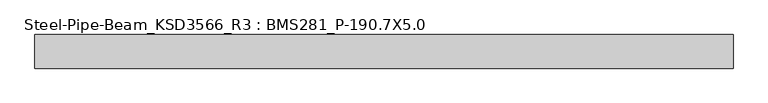
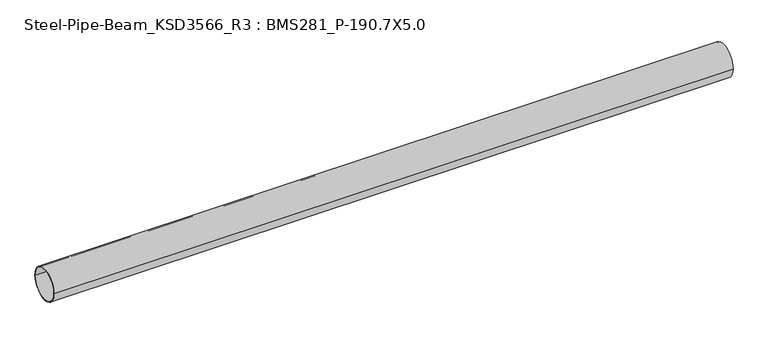
"""IFC4 building model written with IfcOpenShell, lengths in millimetres: member geometry, Steel-Pipe-Beam_KSD3566_R3 : BMS281_P-190.7X5.0."""

from ifc_helpers import new_model, si_unit, point, frame, origin, origin_2d, place, context, project, spatial, circle_curve, trimmed, segment, composite_curve, outline, extrude, source, transform, mapped, element, save


def steel_pipe_beam_ksd3566_r3_bms281_p_190_7x5_0_5ac57b06(model_context):
    return source(origin(), model_context, "Body", "SweptSolid", [
        extrude(outline(composite_curve([segment(trimmed(circle_curve(origin_2d(), 95.35), [point((-95.35, 0.0))], [point((95.35, 0.0))], False, "CARTESIAN"), True, "CONTINUOUS"), segment(trimmed(circle_curve(origin_2d(), 95.35), [point((95.35, 0.0))], [point((-95.35, 0.0))], False, "CARTESIAN"), True, "CONTINUOUS")], self_intersect=False), holes=[composite_curve([segment(trimmed(circle_curve(origin_2d(), 90.35), [point((90.35, 0.0))], [point((-90.35, 0.0))], True, "CARTESIAN"), True, "CONTINUOUS"), segment(trimmed(circle_curve(origin_2d(), 90.35), [point((-90.35, 0.0))], [point((90.35, 0.0))], True, "CARTESIAN"), True, "CONTINUOUS")], self_intersect=False)]), frame((-1988.5748, 0.0, 0.0), z_axis=(1.0, 0.0, 0.0), x_axis=(0.0, 1.0, 0.0)), (0.0, 0.0, 1.0), 3954.0532033),
    ])


if __name__ == "__main__":
    model = new_model("IFC4")
    model_context = context("Model", 3, world=origin())
    ifc_project = project(units=[si_unit("LENGTHUNIT", "METRE", prefix="MILLI")], contexts=[model_context])
    site = spatial("IfcSite", under=ifc_project)
    building = spatial("IfcBuilding", under=site)
    placement = place(None, origin())
    steel_pipe_beam_ksd3566_r3_bms281_p_190_7x5_0_shape = steel_pipe_beam_ksd3566_r3_bms281_p_190_7x5_0_5ac57b06(model_context)
    element("IfcMember", 1, ObjectType="Steel-Pipe-Beam_KSD3566_R3 : BMS281_P-190.7X5.0", at=placement, inside=building, context=model_context, shape_type="MappedRepresentation", body=[
        mapped(steel_pipe_beam_ksd3566_r3_bms281_p_190_7x5_0_shape, transform((0.0, 0.0, 0.0), x_axis=(1.0, 0.0, 0.0), y_axis=(0.0, 1.0, 0.0), z_axis=(0.0, 0.0, 1.0))),
    ])
    save(model, "model.ifc")

# Revit data of these elements
# Type "Steel-Pipe-Beam_KSD3566_R3 : BMS281_P-190.7X5.0"
#   Keynote = "P-190.7X5.0"
#   SteelWeight = "Light"
#   t = 0.0050 m
#   Surface Area = 0.599102 m²/m
#   Section Area = 29.1697 cm²
#   Mass per Unit Length = 22.8982 kg/m
#   Length [instance default] = 1.5000 m
#   D = 0.1907 m
#   hec_material4 [instance default] = none
#   hec_material3 [instance default] = none
#   hec_material2 [instance default] = none
#   hec_material1 [instance default] = none
#   Structural Material [instance default] = Steel, 45-345
#   Assembly Code = ""
# Element 1 (IfcMember, "Steel-Pipe-Beam_KSD3566_R3 : BMS281_P-190.7X5.0")
#   Structural Material = none
# Materials
#   "Steel, 45-345": class "Metal", colour RGB 189 187 185, transparency 0, Description = "Steel 345 MPa", Cost = 0
